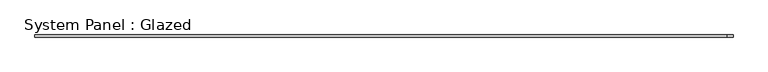
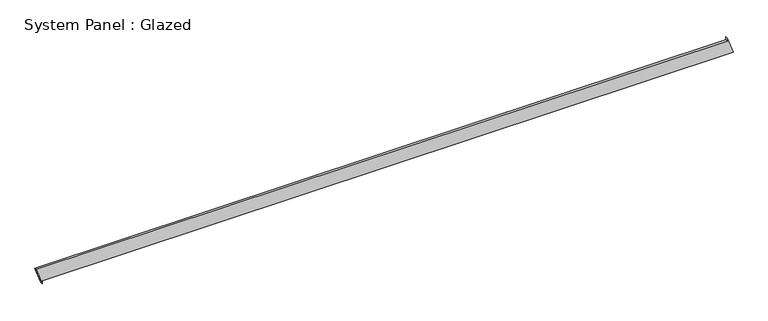
"""IFC4 building model written with IfcOpenShell, lengths in millimetres: plate geometry, System Panel : Glazed."""

from ifc_helpers import new_model, si_unit, frame, origin, place, context, project, spatial, polyline, outline, extrude, source, transform, mapped, element, save


def system_panel_glazed_ce91f84a(model_context):
    return source(origin(), model_context, "Body", "SweptSolid", [
        extrude(outline(polyline([(0.0, -3958.544175), (35.3553391, -3958.544175), (35.3553391, 4027.9549227), (234.4222112, 3958.4885806), (199.0668722, 3958.4884774), (199.0901703, -4027.9549227), (0.0, -3958.544175)])), frame((0.0, -49.5, 0.0), z_axis=(0.0, 1.0, 0.0), x_axis=(0.0, 0.0, 1.0)), (0.0, 0.0, 1.0), 25.0),
    ])


if __name__ == "__main__":
    model = new_model("IFC4")
    model_context = context("Model", 3, world=origin())
    ifc_project = project(units=[si_unit("LENGTHUNIT", "METRE", prefix="MILLI")], contexts=[model_context])
    site = spatial("IfcSite", under=ifc_project)
    building = spatial("IfcBuilding", under=site)
    placement = place(None, origin())
    system_panel_glazed_shape = system_panel_glazed_ce91f84a(model_context)
    element("IfcPlate", 1, ObjectType="System Panel : Glazed", at=placement, inside=building, context=model_context, shape_type="MappedRepresentation", body=[
        mapped(system_panel_glazed_shape, transform((0.0, 0.0, 0.0), x_axis=(1.0, 0.0, 0.0), y_axis=(0.0, 1.0, 0.0), z_axis=(0.0, 0.0, 1.0))),
    ])
    save(model, "model.ifc")

# Revit data of these elements
# Element 1 (IfcPlate, "System Panel : Glazed")
#   Materials on its faces: "Glass"
# Materials
#   "Glass": class "Glass", colour RGB 218 227 224, transparency 0.85, Description = "Soda Lime Glass", Cost = 0
